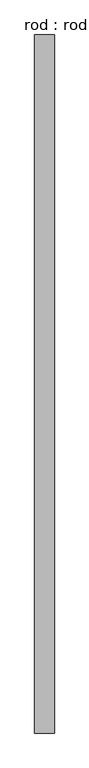
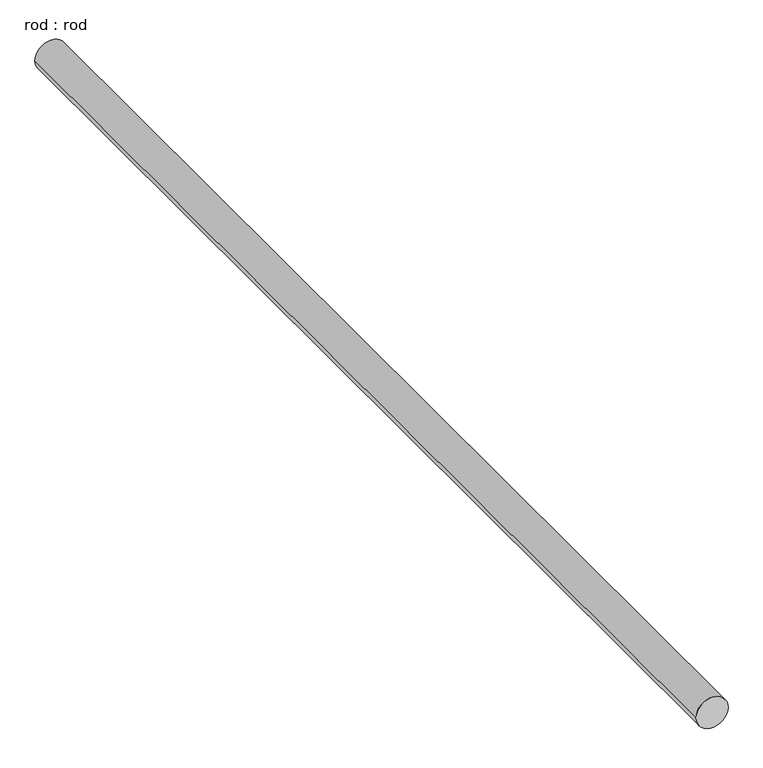
"""IFC4 building model written with IfcOpenShell, lengths in millimetres: proxy geometry, rod : rod."""

from ifc_helpers import new_model, si_unit, point, frame, frame_2d, origin, place, context, project, spatial, circle_curve, trimmed, segment, composite_curve, outline, extrude, source, transform, mapped, element, save


def rod_rod_5a51533f(model_context):
    return source(origin(), model_context, "Body", "SweptSolid", [
        extrude(outline(composite_curve([segment(trimmed(circle_curve(frame_2d((0.0108462, 0.0)), 200.0), [point((0.0108462, 200.0))], [point((0.0108462, -200.0))], False, "CARTESIAN"), True, "CONTINUOUS"), segment(trimmed(circle_curve(frame_2d((0.0108462, 0.0)), 200.0), [point((0.0108462, -200.0))], [point((0.0108462, 200.0))], False, "CARTESIAN"), True, "CONTINUOUS")], self_intersect=False)), frame((0.0, -3030.0907878, 0.0), z_axis=(0.0, 1.0, 0.0), x_axis=(0.0, 0.0, 1.0)), (0.0, 0.0, 1.0), 14245.6388063),
    ])


if __name__ == "__main__":
    model = new_model("IFC4")
    model_context = context("Model", 3, world=origin())
    ifc_project = project(units=[si_unit("LENGTHUNIT", "METRE", prefix="MILLI")], contexts=[model_context])
    site = spatial("IfcSite", under=ifc_project)
    building = spatial("IfcBuilding", under=site)
    placement = place(None, origin())
    rod_rod_shape = rod_rod_5a51533f(model_context)
    element("IfcBuildingElementProxy", 1, Name="rod : rod", ObjectType="rod : rod", at=placement, inside=building, context=model_context, shape_type="MappedRepresentation", body=[
        mapped(rod_rod_shape, transform((0.0, 0.0, 0.0), x_axis=(1.0, 0.0, 0.0), y_axis=(0.0, 1.0, 0.0), z_axis=(0.0, 0.0, 1.0))),
    ])
    save(model, "model.ifc")

# Revit data of these elements
# Type "rod : rod"
#   Default Elevation = 0
